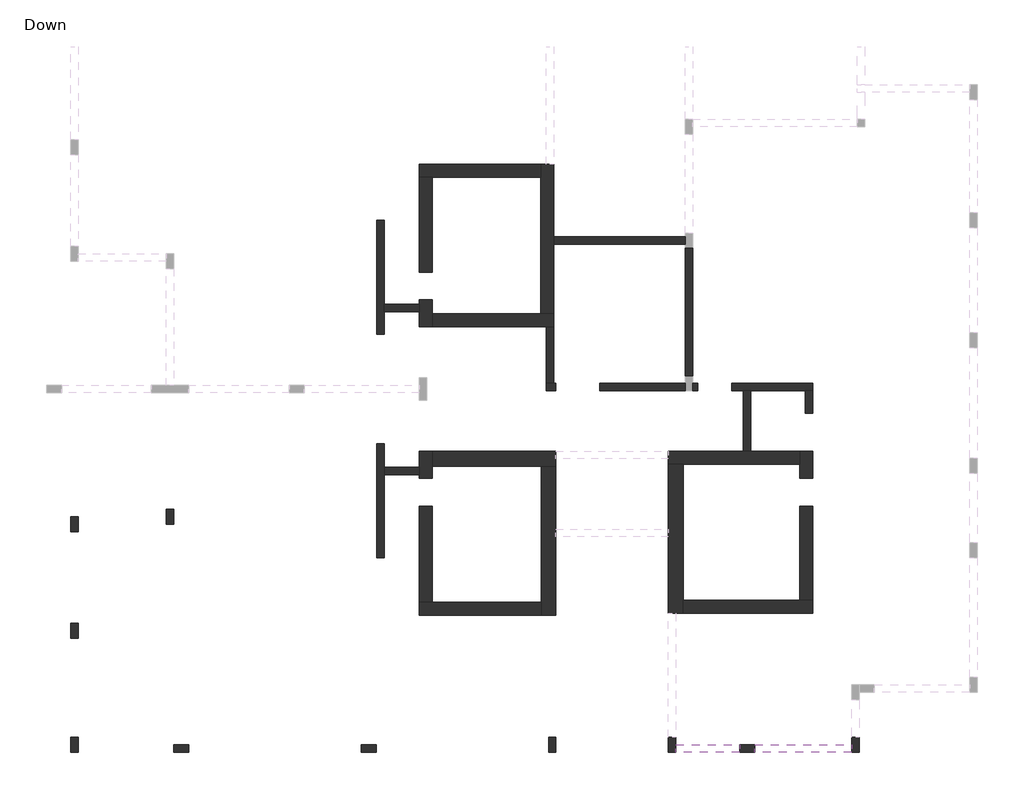
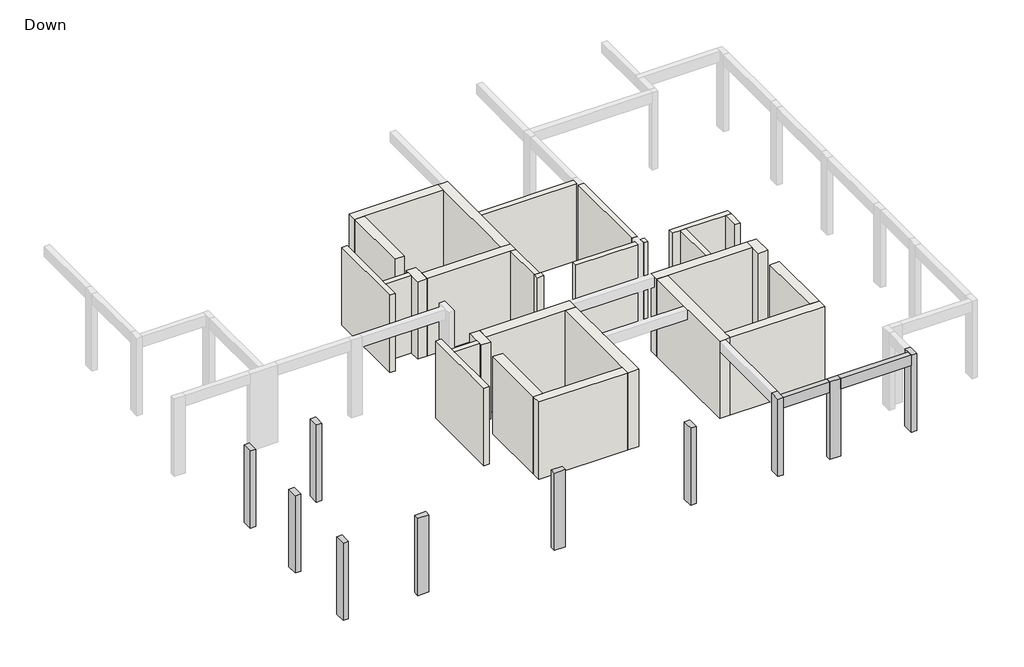
# One storey, part 1 of 2: 28 walls, 10 columns, 2 beams.
"""IFC4 building model written with IfcOpenShell, lengths in millimetres."""

from ifc_helpers import new_model, si_unit, origin, origin_with_axes, place, context, project, spatial, polyline, outline, extrude, faceted_brep, element, save

model = new_model("IFC4")

# Units and contexts
model_context = context("Model", 3, world=origin())
ifc_project = project(units=[si_unit("LENGTHUNIT", "METRE", prefix="MILLI")], contexts=[model_context])

# Site, building, storey
site = spatial("IfcSite", under=ifc_project)
building = spatial("IfcBuilding", under=site)
storey = spatial("IfcBuildingStorey", under=building, Name="Down", Elevation=0.0)

# Beams
placement = place(None, origin())
element("IfcBeam", 1, ObjectType="Concrete Rectengular Beam : 20/40", at=placement, inside=storey, context=model_context, shape_type="Brep", body=[
    faceted_brep([(4052.6741008, -8286.1299304, 3000.0), (4052.6741008, -8486.1299304, 3000.0), (5752.5819696, -8486.1299304, 3000.0), (5752.5819696, -8286.1299304, 3000.0), (4052.6741008, -8286.1299304, 2600.0), (4052.6741008, -8286.1299304, 2780.0), (5752.5819696, -8286.1299304, 2600.0), (4052.6741008, -8486.1299304, 2600.0), (5752.5819696, -8486.1299304, 2600.0)], [[[0, 1, 2, 3]], [[4, 5, 0, 3, 6]], [[7, 4, 6, 8]], [[1, 7, 8, 2]], [[1, 0, 5, 4, 7]], [[3, 2, 8, 6]]]),
])
element("IfcBeam", 2, ObjectType="Concrete Rectengular Beam : 20/40", at=placement, inside=storey, context=model_context, shape_type="Brep", body=[
    faceted_brep([(6152.5819696, -8286.1299304, 3000.0), (6152.5819696, -8486.1299304, 3000.0), (8746.3765637, -8486.1299304, 3000.0), (8746.3765637, -8286.1299304, 3000.0), (6152.5819696, -8486.1299304, 2600.0), (8746.3765637, -8486.1299304, 2600.0), (6152.5819696, -8286.1299304, 2600.0), (8746.3765637, -8286.1299304, 2600.0), (8746.3765637, -8286.1299304, 2780.0)], [[[0, 1, 2, 3]], [[1, 4, 5, 2]], [[4, 6, 7, 5]], [[6, 0, 3, 8, 7]], [[1, 0, 6, 4]], [[3, 2, 5, 7, 8]]]),
])

# Columns
element("IfcColumn", 3, ObjectType="Concrete Rectengular Column : 20/40", at=placement, inside=storey, context=model_context, shape_type="Brep", body=[
    faceted_brep([(-11896.6244933, -8486.1299304, 0.0), (-12096.6244933, -8486.1299304, 0.0), (-12096.6244933, -8086.1299304, 0.0), (-11896.6244933, -8086.1299304, 0.0), (-11896.6244933, -8486.1299304, 3000.0), (-11896.6244933, -8086.1299304, 3000.0), (-11896.6244933, -8286.1299304, 3000.0), (-12096.6244933, -8086.1299304, 3000.0), (-12096.6244933, -8486.1299304, 3000.0)], [[[0, 1, 2, 3]], [[4, 0, 3, 5, 6]], [[5, 3, 2, 7]], [[7, 2, 1, 8]], [[8, 1, 0, 4]], [[4, 6, 5, 7, 8]]]),
])
element("IfcColumn", 4, ObjectType="Concrete Rectengular Column : 20/40", at=placement, inside=storey, context=model_context, shape_type="SweptSolid", body=[
    extrude(outline(polyline([(-9352.4882749, -8486.1299304), (-9352.4882749, -8286.1299304), (-8952.4882749, -8286.1299304), (-8952.4882749, -8486.1299304), (-9352.4882749, -8486.1299304)])), origin_with_axes(), (0.0, 0.0, 1.0), 3000.0),
])
element("IfcColumn", 5, ObjectType="Concrete Rectengular Column : 20/40", at=placement, inside=storey, context=model_context, shape_type="SweptSolid", body=[
    extrude(outline(polyline([(-4346.8056177, -8486.1299304), (-4346.8056177, -8286.1299304), (-3946.8056177, -8286.1299304), (-3946.8056177, -8486.1299304), (-4346.8056177, -8486.1299304)])), origin_with_axes(), (0.0, 0.0, 1.0), 3000.0),
])
element("IfcColumn", 6, ObjectType="Concrete Rectengular Column : 20/40", at=placement, inside=storey, context=model_context, shape_type="Brep", body=[
    faceted_brep([(652.6741008, -8086.1299304, 0.0), (852.6741008, -8086.1299304, 0.0), (852.6741008, -8486.1299304, 0.0), (652.6741008, -8486.1299304, 0.0), (652.6741008, -8086.1299304, 3000.0), (652.6741008, -8486.1299304, 3000.0), (652.6741008, -8286.1299304, 3000.0), (852.6741008, -8486.1299304, 3000.0), (852.6741008, -8086.1299304, 3000.0)], [[[0, 1, 2, 3]], [[4, 0, 3, 5, 6]], [[5, 3, 2, 7]], [[7, 2, 1, 8]], [[8, 1, 0, 4]], [[4, 6, 5, 7, 8]]]),
])
element("IfcColumn", 7, ObjectType="Concrete Rectengular Column : 20/40", at=placement, inside=storey, context=model_context, shape_type="SweptSolid", body=[
    extrude(outline(polyline([(-12096.6244933, -5048.6194614), (-11896.6244933, -5048.6194614), (-11896.6244933, -5448.6194614), (-12096.6244933, -5448.6194614), (-12096.6244933, -5048.6194614)])), origin_with_axes(), (0.0, 0.0, 1.0), 3000.0),
])
element("IfcColumn", 8, ObjectType="Concrete Rectengular Column : 20/40", at=placement, inside=storey, context=model_context, shape_type="Brep", body=[
    faceted_brep([(-12096.6244933, -2198.4826712, 0.0), (-11896.6244933, -2198.4826712, 0.0), (-11896.6244933, -2598.4826712, 0.0), (-12096.6244933, -2598.4826712, 0.0), (-12096.6244933, -2198.4826712, 3000.0), (-12096.6244933, -2598.4826712, 3000.0), (-11896.6244933, -2598.4826712, 3000.0), (-11896.6244933, -2198.4826712, 3000.0), (-11896.6244933, -2398.4826712, 3000.0)], [[[0, 1, 2, 3]], [[4, 0, 3, 5]], [[5, 3, 2, 6]], [[6, 2, 1, 7, 8]], [[7, 1, 0, 4]], [[4, 5, 6, 8, 7]]]),
])
element("IfcColumn", 9, ObjectType="Concrete Rectengular Column : 20/40", at=placement, inside=storey, context=model_context, shape_type="Brep", body=[
    faceted_brep([(-9554.6843469, -1998.4826712, 0.0), (-9354.6843469, -1998.4826712, 0.0), (-9354.6843469, -2398.4826712, 0.0), (-9554.6843469, -2398.4826712, 0.0), (-9554.6843469, -1998.4826712, 3000.0), (-9554.6843469, -2398.4826712, 3000.0), (-9554.6843469, -2198.4826712, 3000.0), (-9354.6843469, -2398.4826712, 2780.0), (-9354.6843469, -2398.4826712, 3000.0), (-9354.6843469, -1998.4826712, 3000.0)], [[[0, 1, 2, 3]], [[4, 0, 3, 5, 6]], [[5, 3, 2, 7, 8]], [[8, 7, 2, 1, 9]], [[9, 1, 0, 4]], [[4, 6, 5, 8, 9]]]),
])
element("IfcColumn", 10, ObjectType="Concrete Rectengular Column : 20/40", at=placement, inside=storey, context=model_context, shape_type="Brep", body=[
    faceted_brep([(4052.6741008, -8086.1299304, 0.0), (4052.6741008, -8486.1299304, 0.0), (3852.6741008, -8486.1299304, 0.0), (3852.6741008, -8086.1299304, 0.0), (4052.6741008, -8086.1299304, 3000.0), (4052.6741008, -8286.1299304, 3000.0), (4052.6741008, -8486.1299304, 3000.0), (3852.6741008, -8486.1299304, 3000.0), (3852.6741008, -8086.1299304, 3000.0)], [[[0, 1, 2, 3]], [[4, 5, 6, 1, 0]], [[6, 7, 2, 1]], [[7, 8, 3, 2]], [[8, 4, 0, 3]], [[4, 8, 7, 6, 5]]]),
])
element("IfcColumn", 11, ObjectType="Concrete Rectengular Column : 20/40", at=placement, inside=storey, context=model_context, shape_type="SweptSolid", body=[
    extrude(outline(polyline([(5752.5819696, -8286.1299304), (6152.5819696, -8286.1299304), (6152.5819696, -8486.1299304), (5752.5819696, -8486.1299304), (5752.5819696, -8286.1299304)])), origin_with_axes(), (0.0, 0.0, 1.0), 3000.0),
])
element("IfcColumn", 12, ObjectType="Concrete Rectengular Column : 20/40", at=placement, inside=storey, context=model_context, shape_type="Brep", body=[
    faceted_brep([(8746.3765637, -8486.1299304, 0.0), (8746.3765637, -8086.1299304, 0.0), (8946.3765637, -8086.1299304, 0.0), (8946.3765637, -8486.1299304, 0.0), (8746.3765637, -8486.1299304, 3000.0), (8746.3765637, -8286.1299304, 3000.0), (8746.3765637, -8086.1299304, 3000.0), (8946.3765637, -8086.1299304, 3000.0), (8946.3765637, -8486.1299304, 3000.0)], [[[0, 1, 2, 3]], [[4, 5, 6, 1, 0]], [[6, 7, 2, 1]], [[7, 8, 3, 2]], [[8, 4, 0, 3]], [[4, 8, 7, 6, 5]]]),
])

# Walls
element("IfcWall", 13, ObjectType="20", at=placement, inside=storey, context=model_context, shape_type="Brep", body=[
    faceted_brep([(-3937.2404282, 5714.0630881, 0.0), (-3937.2404282, 2665.7744518, 0.0), (-3937.2404282, 2665.7744518, 2780.0), (-3937.2404282, 2665.7744518, 3000.0), (-3937.2404282, 5714.0630881, 3000.0), (-3737.2404282, 5714.0630881, 0.0), (-3737.2404282, 5714.0630881, 3000.0), (-3737.2404282, 3468.2359353, 3000.0), (-3737.2404282, 3268.2359353, 3000.0), (-3737.2404282, 2665.7744518, 3000.0), (-3737.2404282, 2665.7744518, 2780.0), (-3737.2404282, 2665.7744518, 0.0), (-3737.2404282, 3268.2359353, 0.0), (-3737.2404282, 3468.2359353, 0.0)], [[[0, 1, 2, 3, 4]], [[5, 6, 7, 8, 9, 10, 11, 12, 13]], [[1, 0, 5, 13, 12, 11]], [[3, 2, 1, 11, 10, 9]], [[4, 3, 9, 8, 7, 6]], [[0, 4, 6, 5]]]),
])
element("IfcWall", 14, ObjectType="20", at=placement, inside=storey, context=model_context, shape_type="Brep", body=[
    faceted_brep([(-3737.2404282, 3268.2359353, 0.0), (-2802.3258992, 3268.2359353, 0.0), (-2802.3258992, 3268.2359353, 2780.0), (-2802.3258992, 3268.2359353, 3000.0), (-3737.2404282, 3268.2359353, 3000.0), (-3737.2404282, 3268.2359353, 2780.0), (-3737.2404282, 3468.2359353, 0.0), (-3737.2404282, 3468.2359353, 2780.0), (-3737.2404282, 3468.2359353, 3000.0), (-2802.3258992, 3468.2359353, 3000.0), (-2802.3258992, 3468.2359353, 2780.0), (-2802.3258992, 3468.2359353, 0.0)], [[[0, 1, 2, 3, 4, 5]], [[6, 7, 8, 9, 10, 11]], [[1, 0, 6, 11]], [[4, 3, 9, 8]], [[0, 5, 4, 8, 7, 6]], [[3, 2, 1, 11, 10, 9]]]),
])
element("IfcWall", 15, ObjectType="20", at=placement, inside=storey, context=model_context, shape_type="Brep", body=[
    faceted_brep([(-3737.2404282, -3300.3155508, 0.0), (-3737.2404282, -1084.488398, 0.0), (-3737.2404282, -884.488398, 0.0), (-3737.2404282, -252.0269144, 0.0), (-3737.2404282, -252.0269144, 2780.0), (-3737.2404282, -252.0269144, 3000.0), (-3737.2404282, -884.488398, 3000.0), (-3737.2404282, -1084.488398, 3000.0), (-3737.2404282, -3300.3155508, 3000.0), (-3937.2404282, -3300.3155508, 0.0), (-3937.2404282, -3300.3155508, 3000.0), (-3937.2404282, -252.0269144, 3000.0), (-3937.2404282, -252.0269144, 2780.0), (-3937.2404282, -252.0269144, 0.0)], [[[0, 1, 2, 3, 4, 5, 6, 7, 8]], [[9, 10, 11, 12, 13]], [[3, 2, 1, 0, 9, 13]], [[5, 4, 3, 13, 12, 11]], [[8, 7, 6, 5, 11, 10]], [[0, 8, 10, 9]]]),
])
element("IfcWall", 16, ObjectType="20", at=placement, inside=storey, context=model_context, shape_type="Brep", body=[
    faceted_brep([(-3737.2404282, -1084.488398, 0.0), (-2802.3258992, -1084.488398, 0.0), (-2802.3258992, -1084.488398, 2780.0), (-2802.3258992, -1084.488398, 3000.0), (-3737.2404282, -1084.488398, 3000.0), (-3737.2404282, -1084.488398, 2780.0), (-3737.2404282, -884.488398, 0.0), (-3737.2404282, -884.488398, 2780.0), (-3737.2404282, -884.488398, 3000.0), (-2802.3258992, -884.488398, 3000.0), (-2802.3258992, -884.488398, 2780.0), (-2802.3258992, -884.488398, 0.0)], [[[0, 1, 2, 3, 4, 5]], [[6, 7, 8, 9, 10, 11]], [[1, 0, 6, 11]], [[4, 3, 9, 8]], [[0, 5, 4, 8, 7, 6]], [[3, 2, 1, 11, 10, 9]]]),
])
element("IfcWall", 17, ObjectType="20", at=placement, inside=storey, context=model_context, shape_type="Brep", body=[
    faceted_brep([(6043.815032, -454.488398, 0.0), (6043.815032, 1157.9050688, 0.0), (6043.815032, 1157.9050688, 2780.0), (6043.815032, 1157.9050688, 3000.0), (6043.815032, -454.488398, 3000.0), (6043.815032, -454.488398, 2780.0), (5843.815032, -454.488398, 0.0), (5843.815032, -454.488398, 2780.0), (5843.815032, -454.488398, 3000.0), (5843.815032, 1157.9050688, 3000.0), (5843.815032, 1157.9050688, 2780.0), (5843.815032, 1157.9050688, 0.0)], [[[0, 1, 2, 3, 4, 5]], [[6, 7, 8, 9, 10, 11]], [[1, 0, 6, 11]], [[4, 3, 9, 8]], [[0, 5, 4, 8, 7, 6]], [[3, 2, 1, 11, 10, 9]]]),
])
element("IfcWall", 18, ObjectType="20", at=placement, inside=storey, context=model_context, shape_type="Brep", body=[
    faceted_brep([(5543.815032, 1157.9050688, 0.0), (5843.815032, 1157.9050688, 0.0), (6043.815032, 1157.9050688, 0.0), (7503.815032, 1157.9050688, 0.0), (7703.815032, 1157.9050688, 0.0), (7703.815032, 1157.9050688, 3000.0), (7503.815032, 1157.9050688, 3000.0), (6043.815032, 1157.9050688, 3000.0), (5843.815032, 1157.9050688, 3000.0), (5543.815032, 1157.9050688, 3000.0), (5543.815032, 1157.9050688, 2780.0), (5543.815032, 1357.9050688, 0.0), (5543.815032, 1357.9050688, 2780.0), (5543.815032, 1357.9050688, 3000.0), (7703.815032, 1357.9050688, 3000.0), (7703.815032, 1357.9050688, 2780.0), (7703.815032, 1357.9050688, 0.0)], [[[0, 1, 2, 3, 4, 5, 6, 7, 8, 9, 10]], [[11, 12, 13, 14, 15, 16]], [[4, 3, 2, 1, 0, 11, 16]], [[9, 8, 7, 6, 5, 14, 13]], [[0, 10, 9, 13, 12, 11]], [[5, 4, 16, 15, 14]]]),
])
element("IfcWall", 19, ObjectType="20", at=placement, inside=storey, context=model_context, shape_type="Brep", body=[
    faceted_brep([(7503.815032, 1157.9050688, 0.0), (7503.815032, 565.511602, 0.0), (7503.815032, 565.511602, 2780.0), (7503.815032, 565.511602, 3000.0), (7503.815032, 1157.9050688, 3000.0), (7503.815032, 1157.9050688, 2780.0), (7703.815032, 1157.9050688, 0.0), (7703.815032, 1157.9050688, 3000.0), (7703.815032, 565.511602, 3000.0), (7703.815032, 565.511602, 2780.0), (7703.815032, 565.511602, 0.0)], [[[0, 1, 2, 3, 4, 5]], [[6, 7, 8, 9, 10]], [[1, 0, 6, 10]], [[3, 2, 1, 10, 9, 8]], [[4, 3, 8, 7]], [[0, 5, 4, 7, 6]]]),
])
element("IfcWall", 20, ObjectType="20", at=placement, inside=storey, context=model_context, shape_type="Brep", body=[
    faceted_brep([(4640.5760436, 1357.9050688, 3000.0), (4640.5760436, 1357.9050688, 2780.0), (4640.5760436, 1357.9050688, 0.0), (4497.0462143, 1357.9050688, 0.0), (4497.0462143, 1357.9050688, 2780.0), (4497.0462143, 1357.9050688, 3000.0), (4640.5760436, 1157.9050688, 0.0), (4640.5760436, 1157.9050688, 2780.0), (4640.5760436, 1157.9050688, 3000.0), (4497.0462143, 1157.9050688, 3000.0), (4497.0462143, 1157.9050688, 0.0)], [[[0, 1, 2, 3, 4, 5]], [[6, 7, 8, 9, 10]], [[2, 6, 10, 3]], [[8, 0, 5, 9]], [[2, 1, 0, 8, 7, 6]], [[5, 4, 3, 10, 9]]]),
])
element("IfcWall", 21, ObjectType="20", at=placement, inside=storey, context=model_context, shape_type="Brep", body=[
    faceted_brep([(4297.0462143, 1357.9050688, 0.0), (2014.3086194, 1357.9050688, 0.0), (2014.3086194, 1357.9050688, 2780.0), (2014.3086194, 1357.9050688, 3000.0), (4297.0462143, 1357.9050688, 3000.0), (4297.0462143, 1357.9050688, 2780.0), (4297.0462143, 1157.9050688, 0.0), (4297.0462143, 1157.9050688, 3000.0), (2014.3086194, 1157.9050688, 3000.0), (2014.3086194, 1157.9050688, 2780.0), (2014.3086194, 1157.9050688, 0.0)], [[[0, 1, 2, 3, 4, 5]], [[6, 7, 8, 9, 10]], [[1, 0, 6, 10]], [[3, 2, 1, 10, 9, 8]], [[4, 3, 8, 7]], [[0, 5, 4, 7, 6]]]),
])
element("IfcWall", 22, ObjectType="20", at=placement, inside=storey, context=model_context, shape_type="Brep", body=[
    faceted_brep([(842.9874073, 1357.9050688, 0.0), (797.6741008, 1357.9050688, 0.0), (597.6741008, 1357.9050688, 0.0), (597.6741008, 1357.9050688, 3000.0), (797.6741008, 1357.9050688, 3000.0), (842.9874073, 1357.9050688, 3000.0), (842.9874073, 1357.9050688, 2780.0), (842.9874073, 1157.9050688, 0.0), (842.9874073, 1157.9050688, 2780.0), (842.9874073, 1157.9050688, 3000.0), (597.6741008, 1157.9050688, 3000.0), (597.6741008, 1157.9050688, 2780.0), (597.6741008, 1157.9050688, 0.0)], [[[0, 1, 2, 3, 4, 5, 6]], [[7, 8, 9, 10, 11, 12]], [[2, 1, 0, 7, 12]], [[5, 4, 3, 10, 9]], [[0, 6, 5, 9, 8, 7]], [[3, 2, 12, 11, 10]]]),
])
element("IfcWall", 23, ObjectType="20", at=placement, inside=storey, context=model_context, shape_type="Brep", body=[
    faceted_brep([(797.6741008, 1357.9050688, 0.0), (797.6741008, 2868.2359353, 0.0), (797.6741008, 2868.2359353, 3000.0), (797.6741008, 1357.9050688, 3000.0), (797.6741008, 1357.9050688, 2780.0), (597.6741008, 1357.9050688, 0.0), (597.6741008, 1357.9050688, 3000.0), (597.6741008, 2868.2359353, 3000.0), (597.6741008, 2868.2359353, 2780.0), (597.6741008, 2868.2359353, 0.0)], [[[0, 1, 2, 3, 4]], [[5, 6, 7, 8, 9]], [[1, 0, 5, 9]], [[3, 2, 7, 6]], [[0, 4, 3, 6, 5]], [[2, 1, 9, 8, 7]]]),
])
element("IfcWall", 24, ObjectType="20", at=placement, inside=storey, context=model_context, shape_type="SweptSolid", body=[
    extrude(outline(polyline([(4497.0462143, 4964.8955051), (4497.0462143, 1557.9050688), (4297.0462143, 1557.9050688), (4297.0462143, 4964.8955051), (4497.0462143, 4964.8955051)])), origin_with_axes(), (0.0, 0.0, 1.0), 3000.0),
])
element("IfcWall", 25, ObjectType="20", at=placement, inside=storey, context=model_context, shape_type="Brep", body=[
    faceted_brep([(4297.0462143, 5264.8955051, 0.0), (797.6741008, 5264.8955051, 0.0), (797.6741008, 5264.8955051, 3000.0), (4297.0462143, 5264.8955051, 3000.0), (4297.0462143, 5064.8955051, 0.0), (4297.0462143, 5064.8955051, 2780.0), (4297.0462143, 5064.8955051, 3000.0), (797.6741008, 5064.8955051, 3000.0), (797.6741008, 5064.8955051, 2780.0), (797.6741008, 5064.8955051, 0.0)], [[[0, 1, 2, 3]], [[4, 5, 6, 7, 8, 9]], [[1, 0, 4, 9]], [[3, 2, 7, 6]], [[0, 3, 6, 5, 4]], [[2, 1, 9, 8, 7]]]),
])
element("IfcWall", 26, ObjectType="35", at=placement, inside=storey, context=model_context, shape_type="Brep", body=[
    faceted_brep([(-2802.3258992, 3588.2359353, 0.0), (-2802.3258992, 3468.2359353, 0.0), (-2802.3258992, 3268.2359353, 0.0), (-2802.3258992, 2868.2359353, 0.0), (-2802.3258992, 2868.2359353, 2780.0), (-2802.3258992, 2868.2359353, 3000.0), (-2802.3258992, 3268.2359353, 3000.0), (-2802.3258992, 3468.2359353, 3000.0), (-2802.3258992, 3588.2359353, 3000.0), (-2802.3258992, 3588.2359353, 2780.0), (-2452.3258992, 3588.2359353, 0.0), (-2452.3258992, 3588.2359353, 2780.0), (-2452.3258992, 3588.2359353, 3000.0), (-2452.3258992, 3218.2359353, 3000.0), (-2452.3258992, 2868.2359353, 3000.0), (-2452.3258992, 2868.2359353, 0.0), (-2452.3258992, 3218.2359353, 0.0), (-2800.2213409, 2868.2359353, 3000.0), (-2457.3258992, 3588.2359353, 3000.0)], [[[0, 1, 2, 3, 4, 5, 6, 7, 8, 9]], [[10, 11, 12, 13, 14, 15, 16]], [[3, 2, 1, 0, 10, 16, 15]], [[8, 7, 6, 5, 17, 14, 13, 12, 18]], [[0, 9, 8, 18, 12, 11, 10]], [[5, 4, 3, 15, 14, 17]]]),
])
element("IfcWall", 27, ObjectType="35", at=placement, inside=storey, context=model_context, shape_type="Brep", body=[
    faceted_brep([(-2452.3258992, 2868.2359353, 0.0), (597.6741008, 2868.2359353, 0.0), (797.6741008, 2868.2359353, 0.0), (797.6741008, 2868.2359353, 3000.0), (597.6741008, 2868.2359353, 3000.0), (-2452.3258992, 2868.2359353, 3000.0), (-2452.3258992, 3218.2359353, 0.0), (-2452.3258992, 3218.2359353, 2780.0), (-2452.3258992, 3218.2359353, 3000.0), (447.6741008, 3218.2359353, 3000.0), (797.6741008, 3218.2359353, 3000.0), (797.6741008, 3218.2359353, 0.0), (447.6741008, 3218.2359353, 0.0)], [[[0, 1, 2, 3, 4, 5]], [[6, 7, 8, 9, 10, 11, 12]], [[2, 1, 0, 6, 12, 11]], [[5, 4, 3, 10, 9, 8]], [[0, 5, 8, 7, 6]], [[3, 2, 11, 10]]]),
])
element("IfcWall", 28, ObjectType="35", at=placement, inside=storey, context=model_context, shape_type="Brep", body=[
    faceted_brep([(797.6741008, 3218.2359353, 0.0), (797.6741008, 5064.8955051, 0.0), (797.6741008, 5264.8955051, 0.0), (797.6741008, 7208.2359353, 0.0), (797.6741008, 7208.2359353, 3000.0), (797.6741008, 5264.8955051, 3000.0), (797.6741008, 5064.8955051, 3000.0), (797.6741008, 3218.2359353, 3000.0), (447.6741008, 3218.2359353, 0.0), (447.6741008, 3218.2359353, 2780.0), (447.6741008, 3218.2359353, 3000.0), (447.6741008, 6858.2359353, 3000.0), (447.6741008, 7208.2359353, 3000.0), (447.6741008, 7208.2359353, 0.0), (447.6741008, 6858.2359353, 0.0), (792.5229388, 7208.2359353, 3000.0), (592.5229388, 7208.2359353, 3000.0)], [[[0, 1, 2, 3, 4, 5, 6, 7]], [[8, 9, 10, 11, 12, 13, 14]], [[3, 2, 1, 0, 8, 14, 13]], [[7, 6, 5, 4, 15, 16, 12, 11, 10]], [[0, 7, 10, 9, 8]], [[4, 3, 13, 12, 16, 15]]]),
])
element("IfcWall", 29, ObjectType="35", at=placement, inside=storey, context=model_context, shape_type="Brep", body=[
    faceted_brep([(447.6741008, 7208.2359353, 0.0), (-2802.3258992, 7208.2359353, 0.0), (-2802.3258992, 7208.2359353, 2780.0), (-2802.3258992, 7208.2359353, 3000.0), (447.6741008, 7208.2359353, 3000.0), (447.6741008, 6858.2359353, 0.0), (447.6741008, 6858.2359353, 2780.0), (447.6741008, 6858.2359353, 3000.0), (-2452.3258992, 6858.2359353, 3000.0), (-2802.3258992, 6858.2359353, 3000.0), (-2802.3258992, 6858.2359353, 0.0), (-2452.3258992, 6858.2359353, 0.0)], [[[0, 1, 2, 3, 4]], [[5, 6, 7, 8, 9, 10, 11]], [[1, 0, 5, 11, 10]], [[4, 3, 9, 8, 7]], [[0, 4, 7, 6, 5]], [[3, 2, 1, 10, 9]]]),
])
element("IfcWall", 30, ObjectType="35", at=placement, inside=storey, context=model_context, shape_type="Brep", body=[
    faceted_brep([(-2802.3258992, 6858.2359353, 0.0), (-2802.3258992, 4328.2359353, 0.0), (-2802.3258992, 4328.2359353, 2780.0), (-2802.3258992, 4328.2359353, 3000.0), (-2802.3258992, 6858.2359353, 3000.0), (-2452.3258992, 6858.2359353, 0.0), (-2452.3258992, 6858.2359353, 2780.0), (-2452.3258992, 6858.2359353, 3000.0), (-2452.3258992, 4328.2359353, 3000.0), (-2452.3258992, 4328.2359353, 2780.0), (-2452.3258992, 4328.2359353, 0.0), (-2457.3258992, 4328.2359353, 3000.0)], [[[0, 1, 2, 3, 4]], [[5, 6, 7, 8, 9, 10]], [[1, 0, 5, 10]], [[3, 2, 1, 10, 9, 8, 11]], [[4, 3, 11, 8, 7]], [[0, 4, 7, 6, 5]]]),
])
element("IfcWall", 31, ObjectType="35", at=placement, inside=storey, context=model_context, shape_type="Brep", body=[
    faceted_brep([(-2452.3258992, -1174.488398, 0.0), (-2452.3258992, -854.488398, 0.0), (-2452.3258992, -454.488398, 0.0), (-2452.3258992, -454.488398, 3000.0), (-2452.3258992, -854.488398, 3000.0), (-2452.3258992, -1174.488398, 3000.0), (-2452.3258992, -1174.488398, 2780.0), (-2802.3258992, -1174.488398, 0.0), (-2802.3258992, -1174.488398, 2780.0), (-2802.3258992, -1174.488398, 3000.0), (-2802.3258992, -1084.488398, 3000.0), (-2802.3258992, -884.488398, 3000.0), (-2802.3258992, -454.488398, 3000.0), (-2802.3258992, -454.488398, 2780.0), (-2802.3258992, -454.488398, 0.0), (-2802.3258992, -884.488398, 0.0), (-2802.3258992, -1084.488398, 0.0), (-2800.2213409, -454.488398, 3000.0)], [[[0, 1, 2, 3, 4, 5, 6]], [[7, 8, 9, 10, 11, 12, 13, 14, 15, 16]], [[2, 1, 0, 7, 16, 15, 14]], [[5, 4, 3, 17, 12, 11, 10, 9]], [[0, 6, 5, 9, 8, 7]], [[3, 2, 14, 13, 12, 17]]]),
])
element("IfcWall", 32, ObjectType="35", at=placement, inside=storey, context=model_context, shape_type="Brep", body=[
    faceted_brep([(452.6741008, -4484.488398, 0.0), (-2452.3258992, -4484.488398, 0.0), (-2802.3258992, -4484.488398, 0.0), (-2802.3258992, -4484.488398, 3000.0), (-2452.3258992, -4484.488398, 3000.0), (452.6741008, -4484.488398, 3000.0), (452.6741008, -4484.488398, 2780.0), (452.6741008, -4834.488398, 0.0), (452.6741008, -4834.488398, 3000.0), (-2802.3258992, -4834.488398, 3000.0), (-2802.3258992, -4834.488398, 2780.0), (-2802.3258992, -4834.488398, 0.0)], [[[0, 1, 2, 3, 4, 5, 6]], [[7, 8, 9, 10, 11]], [[2, 1, 0, 7, 11]], [[5, 4, 3, 9, 8]], [[0, 6, 5, 8, 7]], [[3, 2, 11, 10, 9]]]),
])
element("IfcWall", 33, ObjectType="35", at=placement, inside=storey, context=model_context, shape_type="Brep", body=[
    faceted_brep([(-2452.3258992, -4484.488398, 0.0), (-2452.3258992, -1914.488398, 0.0), (-2452.3258992, -1914.488398, 2780.0), (-2452.3258992, -1914.488398, 3000.0), (-2452.3258992, -4484.488398, 3000.0), (-2452.3258992, -4484.488398, 2780.0), (-2802.3258992, -4484.488398, 0.0), (-2802.3258992, -4484.488398, 3000.0), (-2802.3258992, -1914.488398, 3000.0), (-2802.3258992, -1914.488398, 2780.0), (-2802.3258992, -1914.488398, 0.0)], [[[0, 1, 2, 3, 4, 5]], [[6, 7, 8, 9, 10]], [[1, 0, 6, 10]], [[3, 2, 1, 10, 9, 8]], [[4, 3, 8, 7]], [[0, 5, 4, 7, 6]]]),
])
element("IfcWall", 34, ObjectType="35", at=placement, inside=storey, context=model_context, shape_type="Brep", body=[
    faceted_brep([(7705.8942254, -1174.488398, 0.0), (7705.8942254, -454.488398, 0.0), (7705.8942254, -454.488398, 2780.0), (7705.8942254, -454.488398, 3000.0), (7705.8942254, -1174.488398, 3000.0), (7705.8942254, -1174.488398, 2780.0), (7355.8942254, -1174.488398, 0.0), (7355.8942254, -1174.488398, 2780.0), (7355.8942254, -1174.488398, 3000.0), (7355.8942254, -804.488398, 3000.0), (7355.8942254, -454.488398, 3000.0), (7355.8942254, -454.488398, 0.0), (7355.8942254, -804.488398, 0.0)], [[[0, 1, 2, 3, 4, 5]], [[6, 7, 8, 9, 10, 11, 12]], [[1, 0, 6, 12, 11]], [[4, 3, 10, 9, 8]], [[0, 5, 4, 8, 7, 6]], [[3, 2, 1, 11, 10]]]),
])
element("IfcWall", 35, ObjectType="35", at=placement, inside=storey, context=model_context, shape_type="Brep", body=[
    faceted_brep([(7355.8942254, -454.488398, 0.0), (6043.815032, -454.488398, 0.0), (5843.815032, -454.488398, 0.0), (3852.6741008, -454.488398, 0.0), (3852.6741008, -454.488398, 2600.0), (3852.6741008, -454.488398, 3000.0), (5843.815032, -454.488398, 3000.0), (6043.815032, -454.488398, 3000.0), (7355.8942254, -454.488398, 3000.0), (7355.8942254, -804.488398, 0.0), (7355.8942254, -804.488398, 2780.0), (7355.8942254, -804.488398, 3000.0), (4252.6741008, -804.488398, 3000.0), (3852.6741008, -804.488398, 3000.0), (3852.6741008, -804.488398, 0.0), (4252.6741008, -804.488398, 0.0), (3852.6741008, -654.488398, 3000.0)], [[[0, 1, 2, 3, 4, 5, 6, 7, 8]], [[9, 10, 11, 12, 13, 14, 15]], [[3, 2, 1, 0, 9, 15, 14]], [[8, 7, 6, 5, 16, 13, 12, 11]], [[0, 8, 11, 10, 9]], [[5, 4, 3, 14, 13, 16]]]),
])
element("IfcWall", 36, ObjectType="35", at=placement, inside=storey, context=model_context, shape_type="Brep", body=[
    faceted_brep([(4252.6741008, -4782.6671723, 0.0), (7705.8942254, -4782.6671723, 0.0), (7705.8942254, -4782.6671723, 2780.0), (7705.8942254, -4782.6671723, 3000.0), (4252.6741008, -4782.6671723, 3000.0), (4252.6741008, -4432.6671723, 0.0), (4252.6741008, -4432.6671723, 2780.0), (4252.6741008, -4432.6671723, 3000.0), (7355.8942254, -4432.6671723, 3000.0), (7705.8942254, -4432.6671723, 3000.0), (7705.8942254, -4432.6671723, 0.0), (7355.8942254, -4432.6671723, 0.0)], [[[0, 1, 2, 3, 4]], [[5, 6, 7, 8, 9, 10, 11]], [[1, 0, 5, 11, 10]], [[4, 3, 9, 8, 7]], [[0, 4, 7, 6, 5]], [[3, 2, 1, 10, 9]]]),
])
element("IfcWall", 37, ObjectType="35", at=placement, inside=storey, context=model_context, shape_type="Brep", body=[
    faceted_brep([(7705.8942254, -4432.6671723, 0.0), (7705.8942254, -1914.488398, 0.0), (7705.8942254, -1914.488398, 2780.0), (7705.8942254, -1914.488398, 3000.0), (7705.8942254, -4432.6671723, 3000.0), (7355.8942254, -4432.6671723, 0.0), (7355.8942254, -4432.6671723, 2780.0), (7355.8942254, -4432.6671723, 3000.0), (7355.8942254, -1914.488398, 3000.0), (7355.8942254, -1914.488398, 2780.0), (7355.8942254, -1914.488398, 0.0)], [[[0, 1, 2, 3, 4]], [[5, 6, 7, 8, 9, 10]], [[1, 0, 5, 10]], [[3, 2, 1, 10, 9, 8]], [[4, 3, 8, 7]], [[0, 4, 7, 6, 5]]]),
])
element("IfcWall", 38, ObjectType="40", at=placement, inside=storey, context=model_context, shape_type="Brep", body=[
    faceted_brep([(-2452.3258992, -854.488398, 0.0), (452.6741008, -854.488398, 0.0), (852.6741008, -854.488398, 0.0), (852.6741008, -854.488398, 3000.0), (452.6741008, -854.488398, 3000.0), (-2452.3258992, -854.488398, 3000.0), (-2452.3258992, -854.488398, 2780.0), (-2452.3258992, -454.488398, 0.0), (-2452.3258992, -454.488398, 3000.0), (852.6741008, -454.488398, 3000.0), (852.6741008, -454.488398, 2600.0), (852.6741008, -454.488398, 0.0), (852.6741008, -654.488398, 3000.0)], [[[0, 1, 2, 3, 4, 5, 6]], [[7, 8, 9, 10, 11]], [[2, 1, 0, 7, 11]], [[5, 4, 3, 12, 9, 8]], [[0, 6, 5, 8, 7]], [[3, 2, 11, 10, 9, 12]]]),
])
element("IfcWall", 39, ObjectType="40", at=placement, inside=storey, context=model_context, shape_type="Brep", body=[
    faceted_brep([(452.6741008, -854.488398, 0.0), (452.6741008, -4484.488398, 0.0), (452.6741008, -4834.488398, 0.0), (452.6741008, -4834.488398, 3000.0), (452.6741008, -4484.488398, 3000.0), (452.6741008, -854.488398, 3000.0), (452.6741008, -854.488398, 2780.0), (852.6741008, -854.488398, 0.0), (852.6741008, -854.488398, 3000.0), (852.6741008, -4834.488398, 3000.0), (852.6741008, -4834.488398, 2600.0), (852.6741008, -4834.488398, 0.0), (652.6741008, -4834.488398, 3000.0)], [[[0, 1, 2, 3, 4, 5, 6]], [[7, 8, 9, 10, 11]], [[2, 1, 0, 7, 11]], [[5, 4, 3, 12, 9, 8]], [[0, 6, 5, 8, 7]], [[3, 2, 11, 10, 9, 12]]]),
])
element("IfcWall", 40, ObjectType="40", at=placement, inside=storey, context=model_context, shape_type="Brep", body=[
    faceted_brep([(3852.6741008, -804.488398, 0.0), (3852.6741008, -4782.6671723, 0.0), (3852.6741008, -4782.6671723, 2600.0), (3852.6741008, -4782.6671723, 3000.0), (3852.6741008, -804.488398, 3000.0), (4252.6741008, -804.488398, 0.0), (4252.6741008, -804.488398, 2780.0), (4252.6741008, -804.488398, 3000.0), (4252.6741008, -4432.6671723, 3000.0), (4252.6741008, -4782.6671723, 3000.0), (4252.6741008, -4782.6671723, 0.0), (4252.6741008, -4432.6671723, 0.0), (4052.6741008, -4782.6671723, 3000.0)], [[[0, 1, 2, 3, 4]], [[5, 6, 7, 8, 9, 10, 11]], [[1, 0, 5, 11, 10]], [[4, 3, 12, 9, 8, 7]], [[0, 4, 7, 6, 5]], [[3, 2, 1, 10, 9, 12]]]),
])

save(model, "model.ifc")

# Revit data of these elements
# Project information
#   Project Issue Date = "Issue Date"
#   Project Status = "Project Status"
#   Client Name = "לקוח"
#   Project Address = "Enter address here"
#   Project Name = "Project 038"
#   Project Number = "מספר פרויקט"
# Type "Concrete Rectengular Beam : 20/40"
#   Keynote = "09000"
#   Length [instance default] = 152.4 cm
#   b = 20 cm
#   h = 40 cm
#   Structural Material [instance default] = Concrete
#   Assembly Code = ""
# Type "Concrete Rectengular Column : 20/40"
#   b = 20 cm
#   h = 40 cm
#   Structural Material [instance default] = Concrete
# Type "20"
#   Layers, outside or top first: 20 cm "Concrete" (function 1)
# Type "35"
#   Layers, outside or top first: 35 cm "Concrete" (function 1)
# Type "40"
#   Layers, outside or top first: 40 cm "Concrete" (function 1)
# Element 1 (IfcBeam, "Concrete Rectengular Beam : 20/40")
#   Comments = ""
#   Mark = "B21"
#   SOFiSTiK_AMG_Comments = ""
#   SOFiSTiK_AMG_Scheduled = yes
#   SOFiSTiK_AMG_Adjusted = yes
#   Structural Material = Concrete
#   Phase Created = New Construction
#   Materials on its faces: "Concrete"
# Element 2 (IfcBeam, "Concrete Rectengular Beam : 20/40")
#   Comments = ""
#   Mark = "B22"
#   SOFiSTiK_AMG_Comments = ""
#   SOFiSTiK_AMG_Scheduled = yes
#   SOFiSTiK_AMG_Adjusted = yes
#   Structural Material = Concrete
#   Phase Created = New Construction
#   Materials on its faces: "Concrete"
# Element 3 (IfcColumn, "Concrete Rectengular Column : 20/40")
#   Comments = ""
#   Mark = "C12"
#   SOFiSTiK_AMG_Comments = ""
#   SOFiSTiK_AMG_Scheduled = yes
#   SOFiSTiK_AMG_Adjusted = yes
#   Structural Material = Concrete
#   Phase Created = New Construction
#   Materials on its faces: "Concrete"
# Element 4 (IfcColumn, "Concrete Rectengular Column : 20/40")
#   Comments = ""
#   Mark = "C13"
#   SOFiSTiK_AMG_Comments = ""
#   SOFiSTiK_AMG_Scheduled = yes
#   SOFiSTiK_AMG_Adjusted = yes
#   Structural Material = Concrete
#   Phase Created = New Construction
#   Materials on its faces: "Concrete"
# Element 5 (IfcColumn, "Concrete Rectengular Column : 20/40")
#   Comments = ""
#   Mark = "C14"
#   SOFiSTiK_AMG_Comments = ""
#   SOFiSTiK_AMG_Scheduled = yes
#   SOFiSTiK_AMG_Adjusted = yes
#   Structural Material = Concrete
#   Phase Created = New Construction
#   Materials on its faces: "Concrete"
# Element 6 (IfcColumn, "Concrete Rectengular Column : 20/40")
#   Comments = ""
#   Mark = "C15"
#   SOFiSTiK_AMG_Comments = ""
#   SOFiSTiK_AMG_Scheduled = yes
#   SOFiSTiK_AMG_Adjusted = yes
#   Structural Material = Concrete
#   Phase Created = New Construction
#   Materials on its faces: "Concrete"
# Element 7 (IfcColumn, "Concrete Rectengular Column : 20/40")
#   Comments = ""
#   Mark = "C16"
#   SOFiSTiK_AMG_Comments = ""
#   SOFiSTiK_AMG_Scheduled = yes
#   SOFiSTiK_AMG_Adjusted = yes
#   Structural Material = Concrete
#   Phase Created = New Construction
#   Materials on its faces: "Concrete"
# Element 8 (IfcColumn, "Concrete Rectengular Column : 20/40")
#   Comments = ""
#   Mark = "C17"
#   SOFiSTiK_AMG_Comments = ""
#   SOFiSTiK_AMG_Scheduled = yes
#   SOFiSTiK_AMG_Adjusted = yes
#   Structural Material = Concrete
#   Phase Created = New Construction
#   Materials on its faces: "Concrete"
# Element 9 (IfcColumn, "Concrete Rectengular Column : 20/40")
#   Comments = ""
#   Mark = "C18"
#   SOFiSTiK_AMG_Comments = ""
#   SOFiSTiK_AMG_Scheduled = yes
#   SOFiSTiK_AMG_Adjusted = yes
#   Structural Material = Concrete
#   Phase Created = New Construction
#   Materials on its faces: "Concrete"
# Element 10 (IfcColumn, "Concrete Rectengular Column : 20/40")
#   Comments = ""
#   Mark = "C19"
#   SOFiSTiK_AMG_Comments = ""
#   SOFiSTiK_AMG_Scheduled = yes
#   SOFiSTiK_AMG_Adjusted = yes
#   Structural Material = Concrete
#   Phase Created = New Construction
#   Materials on its faces: "Concrete"
# Element 11 (IfcColumn, "Concrete Rectengular Column : 20/40")
#   Comments = ""
#   Mark = "C20"
#   SOFiSTiK_AMG_Comments = ""
#   SOFiSTiK_AMG_Scheduled = yes
#   SOFiSTiK_AMG_Adjusted = yes
#   Structural Material = Concrete
#   Phase Created = New Construction
#   Materials on its faces: "Concrete"
# Element 12 (IfcColumn, "Concrete Rectengular Column : 20/40")
#   Comments = ""
#   Mark = "C21"
#   SOFiSTiK_AMG_Comments = ""
#   SOFiSTiK_AMG_Scheduled = yes
#   SOFiSTiK_AMG_Adjusted = yes
#   Structural Material = Concrete
#   Phase Created = New Construction
#   Materials on its faces: "Concrete"
# Element 13 (IfcWall, "20")
#   Comments = ""
#   Mark = "W1"
#   SOFiSTiK_EdgeZones = "W1"
#   SOFiSTiK_AMG_Comments = ""
#   Top Offset = 0 cm
#   Base Offset = 0 cm
#   wall height = 300 cm
#   SOFiSTiK_AMG_Scheduled = yes
#   SOFiSTiK_AMG_Adjusted = yes
#   Phase Created = New Construction
#   Base Constraint = Down
#   Top Constraint = Typical Floor
#   Materials on its faces: "Concrete"
# Element 14 (IfcWall, "20")
#   Comments = ""
#   Mark = "W2"
#   SOFiSTiK_EdgeZones = "W2"
#   SOFiSTiK_AMG_Comments = ""
#   Top Offset = 0 cm
#   Base Offset = 0 cm
#   wall height = 300 cm
#   SOFiSTiK_AMG_Scheduled = yes
#   SOFiSTiK_AMG_Adjusted = yes
#   Phase Created = New Construction
#   Base Constraint = Down
#   Top Constraint = Typical Floor
#   Materials on its faces: "Concrete"
# Element 15 (IfcWall, "20")
#   Comments = ""
#   Mark = "W3"
#   SOFiSTiK_EdgeZones = "W3"
#   SOFiSTiK_AMG_Comments = ""
#   Top Offset = 0 cm
#   Base Offset = 0 cm
#   wall height = 300 cm
#   SOFiSTiK_AMG_Scheduled = yes
#   SOFiSTiK_AMG_Adjusted = yes
#   Phase Created = New Construction
#   Base Constraint = Down
#   Top Constraint = Typical Floor
#   Materials on its faces: "Concrete"
# Element 16 (IfcWall, "20")
#   Comments = ""
#   Mark = "W4"
#   SOFiSTiK_EdgeZones = "W4"
#   SOFiSTiK_AMG_Comments = ""
#   Top Offset = 0 cm
#   Base Offset = 0 cm
#   wall height = 300 cm
#   SOFiSTiK_AMG_Scheduled = yes
#   SOFiSTiK_AMG_Adjusted = yes
#   Phase Created = New Construction
#   Base Constraint = Down
#   Top Constraint = Typical Floor
#   Materials on its faces: "Concrete"
# Element 17 (IfcWall, "20")
#   Comments = ""
#   Mark = "W5"
#   SOFiSTiK_EdgeZones = "W5"
#   SOFiSTiK_AMG_Comments = ""
#   Top Offset = 0 cm
#   Base Offset = 0 cm
#   wall height = 300 cm
#   SOFiSTiK_AMG_Scheduled = yes
#   SOFiSTiK_AMG_Adjusted = yes
#   Phase Created = New Construction
#   Base Constraint = Down
#   Top Constraint = Typical Floor
#   Materials on its faces: "Concrete"
# Element 18 (IfcWall, "20")
#   Comments = ""
#   Mark = "W6"
#   SOFiSTiK_EdgeZones = "W6"
#   SOFiSTiK_AMG_Comments = ""
#   Top Offset = 0 cm
#   Base Offset = 0 cm
#   wall height = 300 cm
#   SOFiSTiK_AMG_Scheduled = yes
#   SOFiSTiK_AMG_Adjusted = yes
#   Phase Created = New Construction
#   Base Constraint = Down
#   Top Constraint = Typical Floor
#   Materials on its faces: "Concrete"
# Element 19 (IfcWall, "20")
#   Comments = ""
#   Mark = "W7"
#   SOFiSTiK_EdgeZones = "W7"
#   SOFiSTiK_AMG_Comments = ""
#   Top Offset = 0 cm
#   Base Offset = 0 cm
#   wall height = 300 cm
#   SOFiSTiK_AMG_Scheduled = yes
#   SOFiSTiK_AMG_Adjusted = yes
#   Phase Created = New Construction
#   Base Constraint = Down
#   Top Constraint = Typical Floor
#   Materials on its faces: "Concrete"
# Element 20 (IfcWall, "20")
#   Comments = ""
#   Mark = "W9"
#   SOFiSTiK_EdgeZones = "W8"
#   SOFiSTiK_AMG_Comments = "Too Short /"
#   Top Offset = 0 cm
#   Base Offset = 0 cm
#   wall height = 300 cm
#   SOFiSTiK_AMG_Scheduled = yes
#   SOFiSTiK_AMG_Adjusted = yes
#   Phase Created = New Construction
#   Base Constraint = Down
#   Top Constraint = Typical Floor
#   Materials on its faces: "Concrete"
# Element 21 (IfcWall, "20")
#   Comments = ""
#   Mark = "W10"
#   SOFiSTiK_EdgeZones = "W9"
#   SOFiSTiK_AMG_Comments = ""
#   Top Offset = 0 cm
#   Base Offset = 0 cm
#   wall height = 300 cm
#   SOFiSTiK_AMG_Scheduled = yes
#   SOFiSTiK_AMG_Adjusted = yes
#   Phase Created = New Construction
#   Base Constraint = Down
#   Top Constraint = Typical Floor
#   Materials on its faces: "Concrete"
# Element 22 (IfcWall, "20")
#   Comments = ""
#   Mark = "W11"
#   SOFiSTiK_EdgeZones = "W10"
#   SOFiSTiK_AMG_Comments = ""
#   Top Offset = 0 cm
#   Base Offset = 0 cm
#   wall height = 300 cm
#   SOFiSTiK_AMG_Scheduled = yes
#   SOFiSTiK_AMG_Adjusted = yes
#   Phase Created = New Construction
#   Base Constraint = Down
#   Top Constraint = Typical Floor
#   Materials on its faces: "Concrete"
# Element 23 (IfcWall, "20")
#   Comments = ""
#   Mark = "W12"
#   SOFiSTiK_EdgeZones = "W11"
#   SOFiSTiK_AMG_Comments = ""
#   Top Offset = 0 cm
#   Base Offset = 0 cm
#   wall height = 300 cm
#   SOFiSTiK_AMG_Scheduled = yes
#   SOFiSTiK_AMG_Adjusted = yes
#   Phase Created = New Construction
#   Base Constraint = Down
#   Top Constraint = Typical Floor
#   Materials on its faces: "Concrete"
# Element 24 (IfcWall, "20")
#   Comments = ""
#   Mark = "W13"
#   SOFiSTiK_EdgeZones = "W12"
#   SOFiSTiK_AMG_Comments = ""
#   Top Offset = 0 cm
#   Base Offset = 0 cm
#   wall height = 300 cm
#   SOFiSTiK_AMG_Scheduled = yes
#   SOFiSTiK_AMG_Adjusted = yes
#   Phase Created = New Construction
#   Base Constraint = Down
#   Top Constraint = Typical Floor
#   Materials on its faces: "Concrete"
# Element 25 (IfcWall, "20")
#   Comments = ""
#   Mark = "W14"
#   SOFiSTiK_EdgeZones = "W13"
#   SOFiSTiK_AMG_Comments = ""
#   Top Offset = 0 cm
#   Base Offset = 0 cm
#   wall height = 300 cm
#   SOFiSTiK_AMG_Scheduled = yes
#   SOFiSTiK_AMG_Adjusted = yes
#   Phase Created = New Construction
#   Base Constraint = Down
#   Top Constraint = Typical Floor
#   Materials on its faces: "Concrete"
# Element 26 (IfcWall, "35")
#   Comments = ""
#   Mark = "W15"
#   SOFiSTiK_EdgeZones = "W14"
#   SOFiSTiK_AMG_Comments = ""
#   Top Offset = 0 cm
#   Base Offset = 0 cm
#   wall height = 300 cm
#   SOFiSTiK_AMG_Scheduled = yes
#   SOFiSTiK_AMG_Adjusted = yes
#   Phase Created = New Construction
#   Base Constraint = Down
#   Top Constraint = Typical Floor
#   Materials on its faces: "Concrete"
# Element 27 (IfcWall, "35")
#   Comments = ""
#   Mark = "W16"
#   SOFiSTiK_EdgeZones = "W15"
#   SOFiSTiK_AMG_Comments = ""
#   Top Offset = 0 cm
#   Base Offset = 0 cm
#   wall height = 300 cm
#   SOFiSTiK_AMG_Scheduled = yes
#   SOFiSTiK_AMG_Adjusted = yes
#   Phase Created = New Construction
#   Base Constraint = Down
#   Top Constraint = Typical Floor
#   Materials on its faces: "Concrete"
# Element 28 (IfcWall, "35")
#   Comments = ""
#   Mark = "W17"
#   SOFiSTiK_EdgeZones = "W16"
#   SOFiSTiK_AMG_Comments = ""
#   Top Offset = 0 cm
#   Base Offset = 0 cm
#   wall height = 300 cm
#   SOFiSTiK_AMG_Scheduled = yes
#   SOFiSTiK_AMG_Adjusted = yes
#   Phase Created = New Construction
#   Base Constraint = Down
#   Top Constraint = Typical Floor
#   Materials on its faces: "Concrete"
# Element 29 (IfcWall, "35")
#   Comments = ""
#   Mark = "W18"
#   SOFiSTiK_EdgeZones = "W17"
#   SOFiSTiK_AMG_Comments = ""
#   Top Offset = 0 cm
#   Base Offset = 0 cm
#   wall height = 300 cm
#   SOFiSTiK_AMG_Scheduled = yes
#   SOFiSTiK_AMG_Adjusted = yes
#   Phase Created = New Construction
#   Base Constraint = Down
#   Top Constraint = Typical Floor
#   Materials on its faces: "Concrete"
# Element 30 (IfcWall, "35")
#   Comments = ""
#   Mark = "W19"
#   SOFiSTiK_EdgeZones = "W18"
#   SOFiSTiK_AMG_Comments = ""
#   Top Offset = 0 cm
#   Base Offset = 0 cm
#   wall height = 300 cm
#   SOFiSTiK_AMG_Scheduled = yes
#   SOFiSTiK_AMG_Adjusted = yes
#   Phase Created = New Construction
#   Base Constraint = Down
#   Top Constraint = Typical Floor
#   Materials on its faces: "Concrete"
# Element 31 (IfcWall, "35")
#   Comments = ""
#   Mark = "W21"
#   SOFiSTiK_EdgeZones = "W19"
#   SOFiSTiK_AMG_Comments = ""
#   Top Offset = 0 cm
#   Base Offset = 0 cm
#   wall height = 300 cm
#   SOFiSTiK_AMG_Scheduled = yes
#   SOFiSTiK_AMG_Adjusted = yes
#   Phase Created = New Construction
#   Base Constraint = Down
#   Top Constraint = Typical Floor
#   Materials on its faces: "Concrete"
# Element 32 (IfcWall, "35")
#   Comments = ""
#   Mark = "W22"
#   SOFiSTiK_EdgeZones = "W20"
#   SOFiSTiK_AMG_Comments = ""
#   Top Offset = 0 cm
#   Base Offset = 0 cm
#   wall height = 300 cm
#   SOFiSTiK_AMG_Scheduled = yes
#   SOFiSTiK_AMG_Adjusted = yes
#   Phase Created = New Construction
#   Base Constraint = Down
#   Top Constraint = Typical Floor
#   Materials on its faces: "Concrete"
# Element 33 (IfcWall, "35")
#   Comments = ""
#   Mark = "W23"
#   SOFiSTiK_EdgeZones = "W21"
#   SOFiSTiK_AMG_Comments = ""
#   Top Offset = 0 cm
#   Base Offset = 0 cm
#   wall height = 300 cm
#   SOFiSTiK_AMG_Scheduled = yes
#   SOFiSTiK_AMG_Adjusted = yes
#   Phase Created = New Construction
#   Base Constraint = Down
#   Top Constraint = Typical Floor
#   Materials on its faces: "Concrete"
# Element 34 (IfcWall, "35")
#   Comments = ""
#   Mark = "W25"
#   SOFiSTiK_EdgeZones = "W22"
#   SOFiSTiK_AMG_Comments = ""
#   Top Offset = 0 cm
#   Base Offset = 0 cm
#   wall height = 300 cm
#   SOFiSTiK_AMG_Scheduled = yes
#   SOFiSTiK_AMG_Adjusted = yes
#   Phase Created = New Construction
#   Base Constraint = Down
#   Top Constraint = Typical Floor
#   Materials on its faces: "Concrete"
# Element 35 (IfcWall, "35")
#   Comments = ""
#   Mark = "W26"
#   SOFiSTiK_EdgeZones = "W23"
#   SOFiSTiK_AMG_Comments = ""
#   Top Offset = 0 cm
#   Base Offset = 0 cm
#   wall height = 300 cm
#   SOFiSTiK_AMG_Scheduled = yes
#   SOFiSTiK_AMG_Adjusted = yes
#   Phase Created = New Construction
#   Base Constraint = Down
#   Top Constraint = Typical Floor
#   Materials on its faces: "Concrete"
# Element 36 (IfcWall, "35")
#   Comments = ""
#   Mark = "W27"
#   SOFiSTiK_EdgeZones = "W24"
#   SOFiSTiK_AMG_Comments = ""
#   Top Offset = 0 cm
#   Base Offset = 0 cm
#   wall height = 300 cm
#   SOFiSTiK_AMG_Scheduled = yes
#   SOFiSTiK_AMG_Adjusted = yes
#   Phase Created = New Construction
#   Base Constraint = Down
#   Top Constraint = Typical Floor
#   Materials on its faces: "Concrete"
# Element 37 (IfcWall, "35")
#   Comments = ""
#   Mark = "W28"
#   SOFiSTiK_EdgeZones = "W25"
#   SOFiSTiK_AMG_Comments = ""
#   Top Offset = 0 cm
#   Base Offset = 0 cm
#   wall height = 300 cm
#   SOFiSTiK_AMG_Scheduled = yes
#   SOFiSTiK_AMG_Adjusted = yes
#   Phase Created = New Construction
#   Base Constraint = Down
#   Top Constraint = Typical Floor
#   Materials on its faces: "Concrete"
# Element 38 (IfcWall, "40")
#   Comments = ""
#   Mark = "W30"
#   SOFiSTiK_EdgeZones = "W26"
#   SOFiSTiK_AMG_Comments = ""
#   Top Offset = 0 cm
#   Base Offset = 0 cm
#   wall height = 300 cm
#   SOFiSTiK_AMG_Scheduled = yes
#   SOFiSTiK_AMG_Adjusted = yes
#   Phase Created = New Construction
#   Base Constraint = Down
#   Top Constraint = Typical Floor
#   Materials on its faces: "Concrete"
# Element 39 (IfcWall, "40")
#   Comments = ""
#   Mark = "W31"
#   SOFiSTiK_EdgeZones = "W27"
#   SOFiSTiK_AMG_Comments = ""
#   Top Offset = 0 cm
#   Base Offset = 0 cm
#   wall height = 300 cm
#   SOFiSTiK_AMG_Scheduled = yes
#   SOFiSTiK_AMG_Adjusted = yes
#   Phase Created = New Construction
#   Base Constraint = Down
#   Top Constraint = Typical Floor
#   Materials on its faces: "Concrete"
# Element 40 (IfcWall, "40")
#   Comments = ""
#   Mark = "W32"
#   SOFiSTiK_EdgeZones = "W28"
#   SOFiSTiK_AMG_Comments = ""
#   Top Offset = 0 cm
#   Base Offset = 0 cm
#   wall height = 300 cm
#   SOFiSTiK_AMG_Scheduled = yes
#   SOFiSTiK_AMG_Adjusted = yes
#   Phase Created = New Construction
#   Base Constraint = Down
#   Top Constraint = Typical Floor
#   Materials on its faces: "Concrete"
# Materials
#   "Concrete": class "Concrete", colour RGB 192 192 192, transparency 0, Keynote = "01000", Description = "Cast-in-place concrete", Cost = 0
